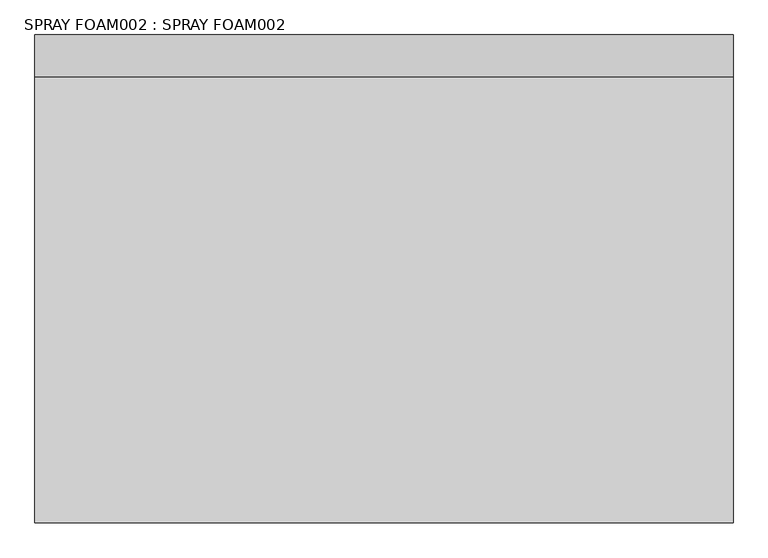
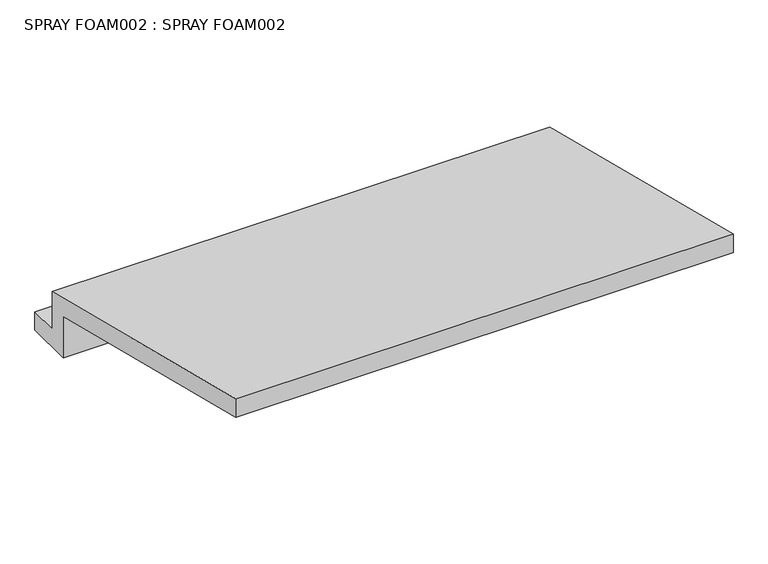
"""IFC4 building model written with IfcOpenShell, lengths in millimetres: proxy geometry, SPRAY FOAM002 : SPRAY FOAM002."""

import ifcopenshell
import ifcopenshell.guid

model = None  # the IFC model being written
_history = None  # IfcOwnerHistory: only IFC2X3 demands one
_inside = {}  # id of a spatial element -> (the spatial element, [elements in it])
_under = {}  # id of a project, library or spatial element -> (it, [spatial elements below it])
_declared = {}  # id of a project -> (the project, [libraries it declares])
_typed = {}  # id of a type object -> (the type object, [elements of that type])
_made_of = {}  # id of a material, layer set ... -> (it, [elements and type objects made of it])


def new_model(schema):
    """Start an empty IFC model of exactly this schema.

    Asked for "IFC4X3", IfcOpenShell would pick the latest addendum, in which some entities
    have other attributes; the version numbers below select the first issue.
    IFC2X3 requires an IfcOwnerHistory on every rooted entity: one is made here for all.
    """
    global model, _history
    if schema == "IFC4X3":
        model = ifcopenshell.file(schema_version=(4, 3, 0, 0))
    else:
        model = ifcopenshell.file(schema=schema)
    _inside.clear()
    _under.clear()
    _declared.clear()
    _typed.clear()
    _made_of.clear()
    _history = None
    if model.schema == "IFC2X3":
        org = make("IfcOrganization", Name="unknown")
        user = make(
            "IfcPersonAndOrganization",
            ThePerson=make("IfcPerson", FamilyName="unknown"),
            TheOrganization=org,
        )
        app = make(
            "IfcApplication",
            ApplicationDeveloper=org,
            Version="unknown",
            ApplicationFullName="unknown",
            ApplicationIdentifier="unknown",
        )
        _history = make(
            "IfcOwnerHistory",
            OwningUser=user,
            OwningApplication=app,
            ChangeAction="ADDED",
            CreationDate=0,
        )
    return model


def make(cls, **values):
    """One entity of the class cls with the attributes given. An attribute that is None is left unset."""
    return model.create_entity(
        cls, **{name: value for name, value in values.items() if value is not None}
    )


def rooted(cls, **values):
    """An entity with a GlobalId (a new one), such as an element, a storey or a relation."""
    return make(cls, GlobalId=ifcopenshell.guid.new(), OwnerHistory=_history, **values)


def si_unit(unit_type, name, prefix=None):
    """IfcSIUnit, for example si_unit("LENGTHUNIT", "METRE", prefix="MILLI")."""
    return make("IfcSIUnit", UnitType=unit_type, Prefix=prefix, Name=name)


def assignment(units):
    """IfcUnitAssignment: the units of a project."""
    return None if units is None else make("IfcUnitAssignment", Units=units)


def point(xyz):
    """IfcCartesianPoint."""
    return None if xyz is None else make("IfcCartesianPoint", Coordinates=xyz)


def direction(xyz):
    """IfcDirection."""
    return None if xyz is None else make("IfcDirection", DirectionRatios=xyz)


def frame(location, z_axis=None, x_axis=None):
    """IfcAxis2Placement3D, a coordinate frame: its origin and axes. An axis left out is left unset."""
    return make(
        "IfcAxis2Placement3D",
        Location=point(location),
        Axis=direction(z_axis),
        RefDirection=direction(x_axis),
    )


def origin():
    """The frame at (0, 0, 0) with its axes left unset."""
    return frame((0.0, 0.0, 0.0))


def place(relative_to, where):
    """IfcLocalPlacement: puts the frame where relative to a parent placement (None: the world)."""
    return make(
        "IfcLocalPlacement", PlacementRelTo=relative_to, RelativePlacement=where
    )


def context(
    kind, dimensions, precision=None, world=None, true_north=None, identifier=None
):
    """IfcGeometricRepresentationContext, for example the 3D "Model" context."""
    return make(
        "IfcGeometricRepresentationContext",
        ContextIdentifier=identifier,
        ContextType=kind,
        CoordinateSpaceDimension=dimensions,
        Precision=precision,
        WorldCoordinateSystem=world,
        TrueNorth=true_north,
    )


def project(units=None, contexts=None):
    """IfcProject with its units and contexts."""
    return rooted(
        "IfcProject",
        Name="project",
        RepresentationContexts=contexts,
        UnitsInContext=assignment(units),
    )


def spatial(cls, under=None, at=None, **own):
    """A site, building, storey or space (cls), placed at a placement, below another one or the project."""
    s = rooted(cls, ObjectPlacement=at, **own)
    if under is not None:
        _under.setdefault(under.id(), (under, []))[1].append(s)
    return s


def polyline(points):
    """IfcPolyline through the points."""
    return make("IfcPolyline", Points=[point(p) for p in points])


def outline(outer, holes=None, kind="AREA"):
    """IfcArbitraryClosedProfileDef: a profile drawn as a closed curve; with holes, ...WithVoids."""
    if holes is None:
        return make("IfcArbitraryClosedProfileDef", ProfileType=kind, OuterCurve=outer)
    return make(
        "IfcArbitraryProfileDefWithVoids",
        ProfileType=kind,
        OuterCurve=outer,
        InnerCurves=holes,
    )


def extrude(swept, where, along, depth):
    """IfcExtrudedAreaSolid: the profile swept, set in the frame where, extruded along a direction by depth."""
    return make(
        "IfcExtrudedAreaSolid",
        SweptArea=swept,
        Position=where,
        ExtrudedDirection=direction(along),
        Depth=depth,
    )


def shape(context_of_items, identifier, shape_type, items):
    """IfcShapeRepresentation: the items that make up one representation, for example the "Body"."""
    return make(
        "IfcShapeRepresentation",
        ContextOfItems=context_of_items,
        RepresentationIdentifier=identifier,
        RepresentationType=shape_type,
        Items=items,
    )


def source(mapping_origin, context_of_items, identifier, shape_type, items):
    """IfcRepresentationMap: a shape defined once, which mapped items show again and again."""
    return make(
        "IfcRepresentationMap",
        MappingOrigin=mapping_origin,
        MappedRepresentation=shape(context_of_items, identifier, shape_type, items),
    )


def transform(
    local_origin,
    x_axis=None,
    y_axis=None,
    z_axis=None,
    scale=None,
    scale2=None,
    scale3=None,
    uniform=True,
):
    """IfcCartesianTransformationOperator3D, or its non-uniform kind. x_axis, y_axis, z_axis: its Axis1, 2, 3."""
    if uniform:
        return make(
            "IfcCartesianTransformationOperator3D",
            Axis1=direction(x_axis),
            Axis2=direction(y_axis),
            LocalOrigin=point(local_origin),
            Scale=scale,
            Axis3=direction(z_axis),
        )
    return make(
        "IfcCartesianTransformationOperator3DnonUniform",
        Axis1=direction(x_axis),
        Axis2=direction(y_axis),
        LocalOrigin=point(local_origin),
        Scale=scale,
        Axis3=direction(z_axis),
        Scale2=scale2,
        Scale3=scale3,
    )


def mapped(mapping_source, mapping_target):
    """IfcMappedItem: shows the shape of a source again, moved by a transform."""
    return make(
        "IfcMappedItem", MappingSource=mapping_source, MappingTarget=mapping_target
    )


def made_of(thing, what):
    """Note that an element or type object is made of a material, layer set ...; save() writes the relation."""
    if what is not None:
        _made_of.setdefault(what.id(), (what, []))[1].append(thing)
    return thing


def element(
    cls,
    number,
    at=None,
    inside=None,
    cuts=None,
    type_object=None,
    material=None,
    context=None,
    identifier="Body",
    shape_type=None,
    held_by="IfcProductDefinitionShape",
    body=None,
    shapes=None,
    **own,
):
    """One element of the class cls, such as IfcWall. Its Tag is "e" and its number.

    at: its placement. inside: the storey or other place that contains it. cuts: it is an
    opening in that element (IfcRelVoidsElement). A single representation is given by context,
    identifier, shape_type and body (its items); several are given by shapes. held_by: the class
    of the entity that holds the representations. save() writes the other relations.
    """
    e = rooted(cls, Tag="e%d" % number, ObjectPlacement=at, **own)
    if body is not None:
        shapes = [shape(context, identifier, shape_type, body)]
    if shapes is not None:
        e.Representation = make(held_by, Representations=shapes)
    if inside is not None:
        _inside.setdefault(inside.id(), (inside, []))[1].append(e)
    if cuts is not None:
        rooted(
            "IfcRelVoidsElement", RelatingBuildingElement=cuts, RelatedOpeningElement=e
        )
    if type_object is not None:
        _typed.setdefault(type_object.id(), (type_object, []))[1].append(e)
    return made_of(e, material)


def aggregate(whole, parts):
    """IfcRelAggregates: a whole, such as a stair, and the parts it consists of."""
    return rooted("IfcRelAggregates", RelatingObject=whole, RelatedObjects=parts)


def save(model, path):
    """Write the relations noted so far, then the file.

    IfcRelAggregates (storeys below a building ...), IfcRelContainedInSpatialStructure (elements
    in a storey), IfcRelDefinesByType, IfcRelAssociatesMaterial and IfcRelDeclares: one each for
    every whole, place, type object, material and project.
    """
    for whole, parts in _under.values():
        aggregate(whole, parts)
    for where, things in _inside.values():
        rooted(
            "IfcRelContainedInSpatialStructure",
            RelatedElements=things,
            RelatingStructure=where,
        )
    for kind, things in _typed.values():
        rooted("IfcRelDefinesByType", RelatedObjects=things, RelatingType=kind)
    for what, things in _made_of.values():
        rooted("IfcRelAssociatesMaterial", RelatedObjects=things, RelatingMaterial=what)
    for by, libraries in _declared.values():
        rooted("IfcRelDeclares", RelatingContext=by, RelatedDefinitions=libraries)
    model.write(path)


def spray_foam002_spray_foam002_768a7261(model_context):
    return source(origin(), model_context, "Body", "SweptSolid", [
        extrude(outline(polyline([(4341.3208107, 41477.0623881), (4341.3208107, 41318.4021881), (4461.9707031, 41318.4021881), (4461.9707031, 41242.2021881), (4265.1208107, 41242.2021881), (4265.1208107, 41417.5670859), (3064.132137, 41717.8113414), (3064.132137, 41796.3564587), (4341.3208107, 41477.0623881)])), frame((255.0171875, 0.0, 0.0), z_axis=(1.0, 0.0, 0.0), x_axis=(0.0, 1.0, 0.0)), (0.0, 0.0, 1.0), 1999.85),
    ])


if __name__ == "__main__":
    model = new_model("IFC4")
    model_context = context("Model", 3, world=origin())
    ifc_project = project(units=[si_unit("LENGTHUNIT", "METRE", prefix="MILLI")], contexts=[model_context])
    site = spatial("IfcSite", under=ifc_project)
    building = spatial("IfcBuilding", under=site)
    placement = place(None, origin())
    spray_foam002_spray_foam002_shape = spray_foam002_spray_foam002_768a7261(model_context)
    element("IfcBuildingElementProxy", 1, Name="SPRAY FOAM002 : SPRAY FOAM002", ObjectType="SPRAY FOAM002 : SPRAY FOAM002", at=placement, inside=building, context=model_context, shape_type="MappedRepresentation", body=[
        mapped(spray_foam002_spray_foam002_shape, transform((0.0, 0.0, 0.0), x_axis=(1.0, 0.0, 0.0), y_axis=(0.0, 1.0, 0.0), z_axis=(0.0, 0.0, 1.0))),
    ])
    save(model, "model.ifc")

# Revit data of these elements
# Type "SPRAY FOAM002 : SPRAY FOAM002"
#   NameOverride = "SPRAY FOAM002"
# Element 1 (IfcBuildingElementProxy, "SPRAY FOAM002 : SPRAY FOAM002")
#   Materials on its faces: "POLYURETHANE SPRAY FOAM UNDER ROOF SUBSTRATE (SEE T-24 ENERGY REPORT FOR R-VALUE)"
# Materials
#   "POLYURETHANE SPRAY FOAM UNDER ROOF SUBSTRATE (SEE T-24 ENERGY REPORT FOR R-VALUE)": class "Unassigned", colour RGB 210 164 194, transparency 0, Cost = 0
